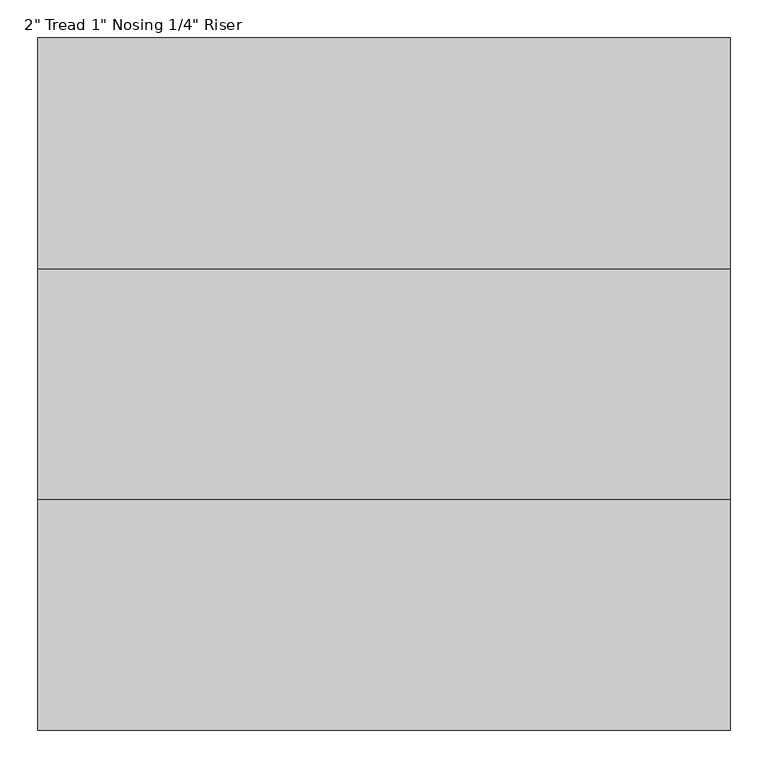
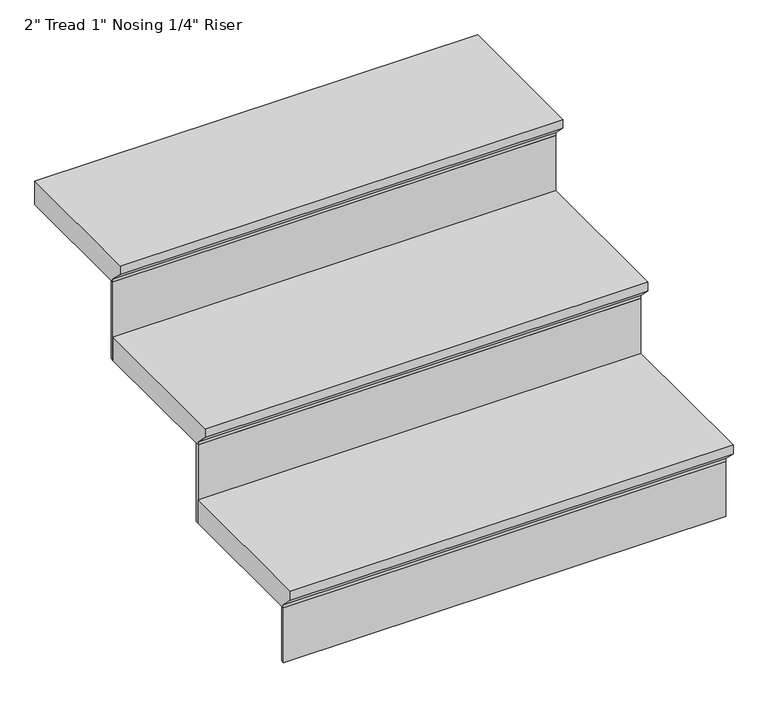
"""IFC4 building model written with IfcOpenShell, lengths in millimetres: stair flight geometry."""

from ifc_helpers import new_model, si_unit, frame, origin, place, context, project, spatial, polyline, outline, extrude, source, transform, mapped, element, save


def stair_flight_a9f6b43f(model_context):
    return source(origin(), model_context, "Body", "SweptSolid", [
        extrude(outline(polyline([(8763.0676078, 1166.6884766), (9093.2676078, 1166.6884766), (9093.2676078, 1115.8884766), (8788.4676078, 1115.8884766), (8788.4676078, 1122.2384766), (8763.0676078, 1147.6384766), (8763.0676078, 1166.6884766)])), frame((-9846.4657498, 0.0, 0.0), z_axis=(1.0, 0.0, 0.0), x_axis=(0.0, 1.0, 0.0)), (0.0, 0.0, 1.0), 914.4),
        extrude(outline(polyline([(-8932.0657498, 8794.8176078), (-8932.0657498, 8788.4676078), (-9846.4657498, 8788.4676078), (-9846.4657498, 8794.8176078), (-8932.0657498, 8794.8176078)])), frame((0.0, 0.0, 995.6601562), z_axis=(0.0, 0.0, 1.0), x_axis=(1.0, 0.0, 0.0)), (0.0, 0.0, 1.0), 120.2283203),
        extrude(outline(polyline([(-8932.0657498, 9099.6176078), (-8932.0657498, 9093.2676078), (-9846.4657498, 9093.2676078), (-9846.4657498, 9099.6176078), (-8932.0657498, 9099.6176078)])), frame((0.0, 0.0, 1115.8884766), z_axis=(0.0, 0.0, 1.0), x_axis=(1.0, 0.0, 0.0)), (0.0, 0.0, 1.0), 171.0283203),
        extrude(outline(polyline([(9067.8676078, 1337.7167969), (9398.0676078, 1337.7167969), (9398.0676078, 1286.9167969), (9093.2676078, 1286.9167969), (9093.2676078, 1293.2667969), (9067.8676078, 1318.6667969), (9067.8676078, 1337.7167969)])), frame((-9846.4657498, 0.0, 0.0), z_axis=(1.0, 0.0, 0.0), x_axis=(0.0, 1.0, 0.0)), (0.0, 0.0, 1.0), 914.4),
        extrude(outline(polyline([(-8932.0657498, 9404.4176078), (-8932.0657498, 9398.0676078), (-9846.4657498, 9398.0676078), (-9846.4657498, 9404.4176078), (-8932.0657498, 9404.4176078)])), frame((0.0, 0.0, 1286.9167969), z_axis=(0.0, 0.0, 1.0), x_axis=(1.0, 0.0, 0.0)), (0.0, 0.0, 1.0), 171.0283203),
        extrude(outline(polyline([(9372.6676078, 1508.7451172), (9677.4676078, 1508.7451172), (9677.4676078, 1457.9451172), (9398.0676078, 1457.9451172), (9398.0676078, 1464.2951172), (9372.6676078, 1489.6951172), (9372.6676078, 1508.7451172)])), frame((-9846.4657498, 0.0, 0.0), z_axis=(1.0, 0.0, 0.0), x_axis=(0.0, 1.0, 0.0)), (0.0, 0.0, 1.0), 914.4),
    ])


if __name__ == "__main__":
    model = new_model("IFC4")
    model_context = context("Model", 3, world=origin())
    ifc_project = project(units=[si_unit("LENGTHUNIT", "METRE", prefix="MILLI")], contexts=[model_context])
    site = spatial("IfcSite", under=ifc_project)
    building = spatial("IfcBuilding", under=site)
    placement = place(None, origin())
    stair_flight_shape = stair_flight_a9f6b43f(model_context)
    element("IfcStairFlight", 1, ObjectType="2\" Tread 1\" Nosing 1/4\" Riser", at=placement, inside=building, context=model_context, shape_type="MappedRepresentation", body=[
        mapped(stair_flight_shape, transform((0.0, 0.0, 0.0), x_axis=(1.0, 0.0, 0.0), y_axis=(0.0, 1.0, 0.0), z_axis=(0.0, 0.0, 1.0))),
    ])
    save(model, "model.ifc")
